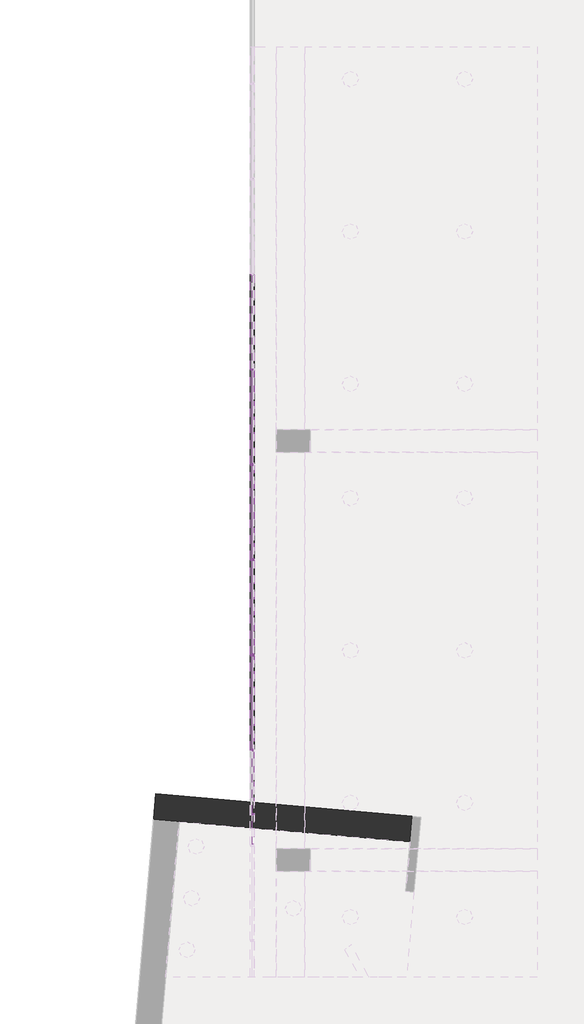
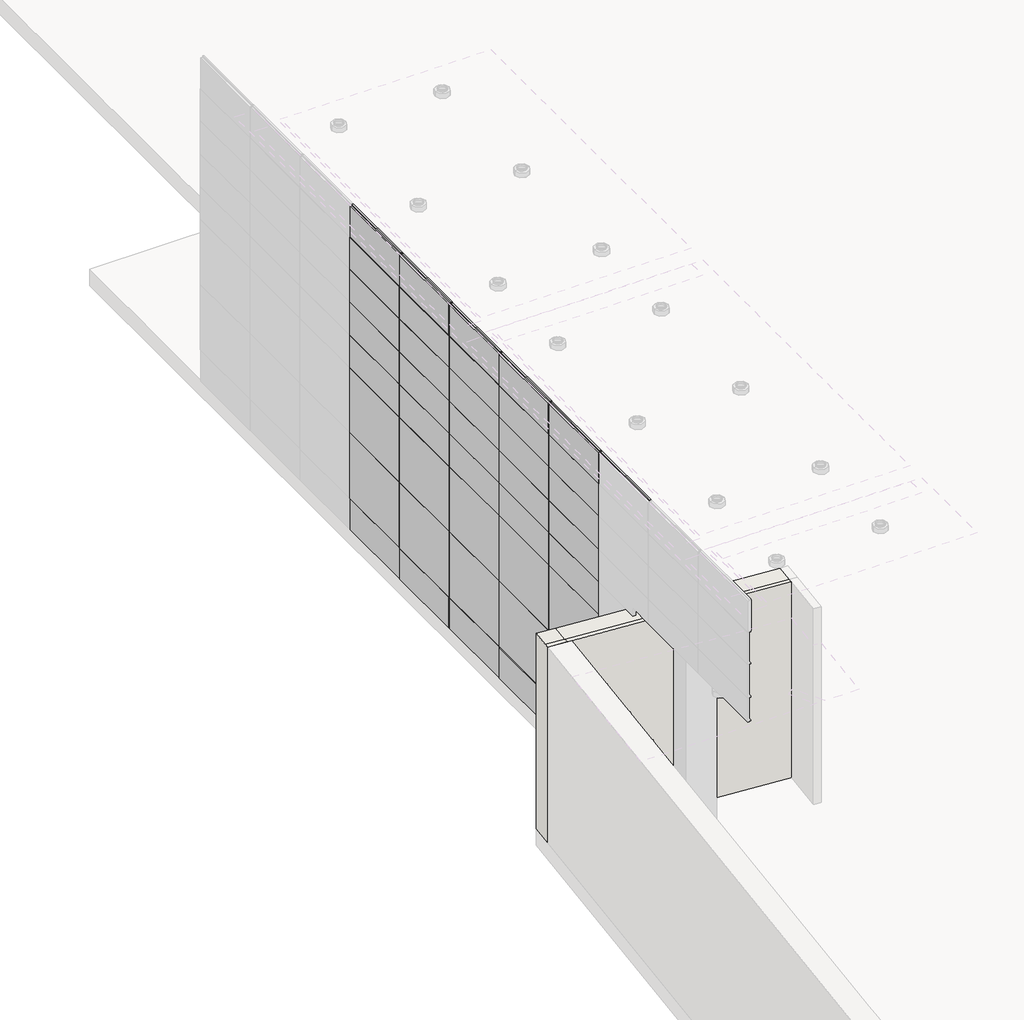
# One storey, part 6 of 30: 90 members, 40 plates, 1 wall.
"""IFC4 building model written with IfcOpenShell, lengths in millimetres."""

import ifcopenshell
import ifcopenshell.guid

model = None  # the IFC model being written
_history = None  # IfcOwnerHistory: only IFC2X3 demands one
_inside = {}  # id of a spatial element -> (the spatial element, [elements in it])
_under = {}  # id of a project, library or spatial element -> (it, [spatial elements below it])
_declared = {}  # id of a project -> (the project, [libraries it declares])
_typed = {}  # id of a type object -> (the type object, [elements of that type])
_made_of = {}  # id of a material, layer set ... -> (it, [elements and type objects made of it])


def new_model(schema):
    """Start an empty IFC model of exactly this schema.

    Asked for "IFC4X3", IfcOpenShell would pick the latest addendum, in which some entities
    have other attributes; the version numbers below select the first issue.
    IFC2X3 requires an IfcOwnerHistory on every rooted entity: one is made here for all.
    """
    global model, _history
    if schema == "IFC4X3":
        model = ifcopenshell.file(schema_version=(4, 3, 0, 0))
    else:
        model = ifcopenshell.file(schema=schema)
    _inside.clear()
    _under.clear()
    _declared.clear()
    _typed.clear()
    _made_of.clear()
    _history = None
    if model.schema == "IFC2X3":
        org = make("IfcOrganization", Name="unknown")
        user = make(
            "IfcPersonAndOrganization",
            ThePerson=make("IfcPerson", FamilyName="unknown"),
            TheOrganization=org,
        )
        app = make(
            "IfcApplication",
            ApplicationDeveloper=org,
            Version="unknown",
            ApplicationFullName="unknown",
            ApplicationIdentifier="unknown",
        )
        _history = make(
            "IfcOwnerHistory",
            OwningUser=user,
            OwningApplication=app,
            ChangeAction="ADDED",
            CreationDate=0,
        )
    return model


def make(cls, **values):
    """One entity of the class cls with the attributes given. An attribute that is None is left unset."""
    return model.create_entity(
        cls, **{name: value for name, value in values.items() if value is not None}
    )


def rooted(cls, **values):
    """An entity with a GlobalId (a new one), such as an element, a storey or a relation."""
    return make(cls, GlobalId=ifcopenshell.guid.new(), OwnerHistory=_history, **values)


def si_unit(unit_type, name, prefix=None):
    """IfcSIUnit, for example si_unit("LENGTHUNIT", "METRE", prefix="MILLI")."""
    return make("IfcSIUnit", UnitType=unit_type, Prefix=prefix, Name=name)


def assignment(units):
    """IfcUnitAssignment: the units of a project."""
    return None if units is None else make("IfcUnitAssignment", Units=units)


def point(xyz):
    """IfcCartesianPoint."""
    return None if xyz is None else make("IfcCartesianPoint", Coordinates=xyz)


def direction(xyz):
    """IfcDirection."""
    return None if xyz is None else make("IfcDirection", DirectionRatios=xyz)


def frame(location, z_axis=None, x_axis=None):
    """IfcAxis2Placement3D, a coordinate frame: its origin and axes. An axis left out is left unset."""
    return make(
        "IfcAxis2Placement3D",
        Location=point(location),
        Axis=direction(z_axis),
        RefDirection=direction(x_axis),
    )


def origin():
    """The frame at (0, 0, 0) with its axes left unset."""
    return frame((0.0, 0.0, 0.0))


def origin_with_axes():
    """The frame at (0, 0, 0) with the z axis (0, 0, 1) and the x axis (1, 0, 0) written out."""
    return frame((0.0, 0.0, 0.0), z_axis=(0.0, 0.0, 1.0), x_axis=(1.0, 0.0, 0.0))


def place(relative_to, where):
    """IfcLocalPlacement: puts the frame where relative to a parent placement (None: the world)."""
    return make(
        "IfcLocalPlacement", PlacementRelTo=relative_to, RelativePlacement=where
    )


def context(
    kind, dimensions, precision=None, world=None, true_north=None, identifier=None
):
    """IfcGeometricRepresentationContext, for example the 3D "Model" context."""
    return make(
        "IfcGeometricRepresentationContext",
        ContextIdentifier=identifier,
        ContextType=kind,
        CoordinateSpaceDimension=dimensions,
        Precision=precision,
        WorldCoordinateSystem=world,
        TrueNorth=true_north,
    )


def project(units=None, contexts=None):
    """IfcProject with its units and contexts."""
    return rooted(
        "IfcProject",
        Name="project",
        RepresentationContexts=contexts,
        UnitsInContext=assignment(units),
    )


def spatial(cls, under=None, at=None, **own):
    """A site, building, storey or space (cls), placed at a placement, below another one or the project."""
    s = rooted(cls, ObjectPlacement=at, **own)
    if under is not None:
        _under.setdefault(under.id(), (under, []))[1].append(s)
    return s


def polyline(points):
    """IfcPolyline through the points."""
    return make("IfcPolyline", Points=[point(p) for p in points])


def outline(outer, holes=None, kind="AREA"):
    """IfcArbitraryClosedProfileDef: a profile drawn as a closed curve; with holes, ...WithVoids."""
    if holes is None:
        return make("IfcArbitraryClosedProfileDef", ProfileType=kind, OuterCurve=outer)
    return make(
        "IfcArbitraryProfileDefWithVoids",
        ProfileType=kind,
        OuterCurve=outer,
        InnerCurves=holes,
    )


def extrude(swept, where, along, depth):
    """IfcExtrudedAreaSolid: the profile swept, set in the frame where, extruded along a direction by depth."""
    return make(
        "IfcExtrudedAreaSolid",
        SweptArea=swept,
        Position=where,
        ExtrudedDirection=direction(along),
        Depth=depth,
    )


def faces_of(points, faces, orient=None, outer=None):
    """IfcFace entities. A face is a list of loops; a loop is a list of indices into points, from 0.

    orient and outer hold one flag for each loop. By default every Orientation is true, the
    first loop of a face is its IfcFaceOuterBound and the others are IfcFaceBound.
    """
    made = []
    for i, loops in enumerate(faces):
        bounds = []
        for j, loop in enumerate(loops):
            is_outer = j == 0 if outer is None else outer[i][j]
            bounds.append(
                make(
                    "IfcFaceOuterBound" if is_outer else "IfcFaceBound",
                    Bound=make("IfcPolyLoop", Polygon=[points[k] for k in loop]),
                    Orientation=True if orient is None else orient[i][j],
                )
            )
        made.append(make("IfcFace", Bounds=bounds))
    return made


def faceted_brep(points, faces, orient=None, outer=None, voids=None):
    """IfcFacetedBrep: a solid bounded by flat faces; with voids (closed shells), ...WithVoids."""
    shared = [point(p) for p in points]
    hull = make("IfcClosedShell", CfsFaces=faces_of(shared, faces, orient, outer))
    if voids is None:
        return make("IfcFacetedBrep", Outer=hull)
    return make(
        "IfcFacetedBrepWithVoids",
        Outer=hull,
        Voids=[
            make(cls, CfsFaces=faces_of(shared, fs, o, b)) for cls, fs, o, b in voids
        ],
    )


def shape(context_of_items, identifier, shape_type, items):
    """IfcShapeRepresentation: the items that make up one representation, for example the "Body"."""
    return make(
        "IfcShapeRepresentation",
        ContextOfItems=context_of_items,
        RepresentationIdentifier=identifier,
        RepresentationType=shape_type,
        Items=items,
    )


def source(mapping_origin, context_of_items, identifier, shape_type, items):
    """IfcRepresentationMap: a shape defined once, which mapped items show again and again."""
    return make(
        "IfcRepresentationMap",
        MappingOrigin=mapping_origin,
        MappedRepresentation=shape(context_of_items, identifier, shape_type, items),
    )


def transform(
    local_origin,
    x_axis=None,
    y_axis=None,
    z_axis=None,
    scale=None,
    scale2=None,
    scale3=None,
    uniform=True,
):
    """IfcCartesianTransformationOperator3D, or its non-uniform kind. x_axis, y_axis, z_axis: its Axis1, 2, 3."""
    if uniform:
        return make(
            "IfcCartesianTransformationOperator3D",
            Axis1=direction(x_axis),
            Axis2=direction(y_axis),
            LocalOrigin=point(local_origin),
            Scale=scale,
            Axis3=direction(z_axis),
        )
    return make(
        "IfcCartesianTransformationOperator3DnonUniform",
        Axis1=direction(x_axis),
        Axis2=direction(y_axis),
        LocalOrigin=point(local_origin),
        Scale=scale,
        Axis3=direction(z_axis),
        Scale2=scale2,
        Scale3=scale3,
    )


def mapped(mapping_source, mapping_target):
    """IfcMappedItem: shows the shape of a source again, moved by a transform."""
    return make(
        "IfcMappedItem", MappingSource=mapping_source, MappingTarget=mapping_target
    )


def made_of(thing, what):
    """Note that an element or type object is made of a material, layer set ...; save() writes the relation."""
    if what is not None:
        _made_of.setdefault(what.id(), (what, []))[1].append(thing)
    return thing


def element(
    cls,
    number,
    at=None,
    inside=None,
    cuts=None,
    type_object=None,
    material=None,
    context=None,
    identifier="Body",
    shape_type=None,
    held_by="IfcProductDefinitionShape",
    body=None,
    shapes=None,
    **own,
):
    """One element of the class cls, such as IfcWall. Its Tag is "e" and its number.

    at: its placement. inside: the storey or other place that contains it. cuts: it is an
    opening in that element (IfcRelVoidsElement). A single representation is given by context,
    identifier, shape_type and body (its items); several are given by shapes. held_by: the class
    of the entity that holds the representations. save() writes the other relations.
    """
    e = rooted(cls, Tag="e%d" % number, ObjectPlacement=at, **own)
    if body is not None:
        shapes = [shape(context, identifier, shape_type, body)]
    if shapes is not None:
        e.Representation = make(held_by, Representations=shapes)
    if inside is not None:
        _inside.setdefault(inside.id(), (inside, []))[1].append(e)
    if cuts is not None:
        rooted(
            "IfcRelVoidsElement", RelatingBuildingElement=cuts, RelatedOpeningElement=e
        )
    if type_object is not None:
        _typed.setdefault(type_object.id(), (type_object, []))[1].append(e)
    return made_of(e, material)


def aggregate(whole, parts):
    """IfcRelAggregates: a whole, such as a stair, and the parts it consists of."""
    return rooted("IfcRelAggregates", RelatingObject=whole, RelatedObjects=parts)


def save(model, path):
    """Write the relations noted so far, then the file.

    IfcRelAggregates (storeys below a building ...), IfcRelContainedInSpatialStructure (elements
    in a storey), IfcRelDefinesByType, IfcRelAssociatesMaterial and IfcRelDeclares: one each for
    every whole, place, type object, material and project.
    """
    for whole, parts in _under.values():
        aggregate(whole, parts)
    for where, things in _inside.values():
        rooted(
            "IfcRelContainedInSpatialStructure",
            RelatedElements=things,
            RelatingStructure=where,
        )
    for kind, things in _typed.values():
        rooted("IfcRelDefinesByType", RelatedObjects=things, RelatingType=kind)
    for what, things in _made_of.values():
        rooted("IfcRelAssociatesMaterial", RelatedObjects=things, RelatingMaterial=what)
    for by, libraries in _declared.values():
        rooted("IfcRelDeclares", RelatingContext=by, RelatedDefinitions=libraries)
    model.write(path)


def member_f4845628(model_context):
    return source(origin(), model_context, "Body", "SweptSolid", [
        extrude(outline(polyline([(12.7, 12.7), (12.7, -12.7), (-12.7, -12.7), (-12.7, 12.7), (12.7, 12.7)])), frame((0.0, 0.0, -1219.2), z_axis=(0.0, 0.0, 1.0), x_axis=(1.0, 0.0, 0.0)), (0.0, 0.0, 1.0), 1219.2),
    ])


def member_6604d1e0(model_context):
    return source(origin(), model_context, "Body", "SweptSolid", [
        extrude(outline(polyline([(0.0, 12.7), (0.0, -12.7), (-25.4, -12.7), (-25.4, 12.7), (0.0, 12.7)])), frame((0.0, 0.0, -1498.6), z_axis=(0.0, 0.0, 1.0), x_axis=(1.0, 0.0, 0.0)), (0.0, 0.0, 1.0), 1498.6),
    ])


def member_68981e21(model_context):
    return source(origin(), model_context, "Body", "SweptSolid", [
        extrude(outline(polyline([(0.0, 12.7), (0.0, -12.7), (-25.4, -12.7), (-25.4, 12.7), (0.0, 12.7)])), frame((0.0, 0.0, -609.6), z_axis=(0.0, 0.0, 1.0), x_axis=(1.0, 0.0, 0.0)), (0.0, 0.0, 1.0), 609.6),
    ])


def member_9fd3d903(model_context):
    return source(origin(), model_context, "Body", "SweptSolid", [
        extrude(outline(polyline([(12.7, 12.7), (12.7, -12.7), (-12.7, -12.7), (-12.7, 12.7), (12.7, 12.7)])), frame((0.0, 0.0, -1498.6), z_axis=(0.0, 0.0, 1.0), x_axis=(1.0, 0.0, 0.0)), (0.0, 0.0, 1.0), 1498.6),
    ])


def member_3e1f1dd8(model_context):
    return source(origin(), model_context, "Body", "SweptSolid", [
        extrude(outline(polyline([(12.7, 12.7), (12.7, -12.7), (-12.7, -12.7), (-12.7, 12.7), (12.7, 12.7)])), frame((0.0, 0.0, -609.6), z_axis=(0.0, 0.0, 1.0), x_axis=(1.0, 0.0, 0.0)), (0.0, 0.0, 1.0), 609.6),
    ])


def member_93cf2621(model_context):
    return source(origin(), model_context, "Body", "SweptSolid", [
        extrude(outline(polyline([(12.7, 12.7), (12.7, -12.7), (-12.7, -12.7), (-12.7, 12.7), (12.7, 12.7)])), frame((0.0, 0.0, -622.3), z_axis=(0.0, 0.0, 1.0), x_axis=(1.0, 0.0, 0.0)), (0.0, 0.0, 1.0), 622.3),
    ])


def member_0acad92b(model_context):
    return source(origin(), model_context, "Body", "SweptSolid", [
        extrude(outline(polyline([(12.7, 12.7), (12.7, -12.7), (-12.7, -12.7), (-12.7, 12.7), (12.7, 12.7)])), frame((0.0, 0.0, -596.9), z_axis=(0.0, 0.0, 1.0), x_axis=(1.0, 0.0, 0.0)), (0.0, 0.0, 1.0), 596.9),
    ])


def member_b874cca0(model_context):
    return source(origin(), model_context, "Body", "SweptSolid", [
        extrude(outline(polyline([(12.7, 12.7), (12.7, -12.7), (-12.7, -12.7), (-12.7, 12.7), (12.7, 12.7)])), frame((0.0, 0.0, -1004.9287927), z_axis=(0.0, 0.0, 1.0), x_axis=(1.0, 0.0, 0.0)), (0.0, 0.0, 1.0), 1004.9287927),
    ])


def system_panel_glazed_327285c7(model_context):
    return source(origin(), model_context, "Body", "SweptSolid", [
        extrude(outline(polyline([(762.0, 19.05), (-762.0, 19.05), (-762.0, 44.45), (762.0, 44.45), (762.0, 19.05)])), origin_with_axes(), (0.0, 0.0, 1.0), 609.6),
    ])


def system_panel_glazed_14200f5a(model_context):
    return source(origin(), model_context, "Body", "SweptSolid", [
        extrude(outline(polyline([(762.0, 19.05), (-762.0, 19.05), (-762.0, 44.45), (762.0, 44.45), (762.0, 19.05)])), origin_with_axes(), (0.0, 0.0, 1.0), 1219.2),
    ])


def system_panel_glazed_39099b5e(model_context):
    return source(origin(), model_context, "Body", "SweptSolid", [
        extrude(outline(polyline([(762.0, 19.05), (-762.0, 19.05), (-762.0, 44.45), (762.0, 44.45), (762.0, 19.05)])), origin_with_axes(), (0.0, 0.0, 1.0), 622.3),
    ])


def system_panel_glazed_72237fa4(model_context):
    return source(origin(), model_context, "Body", "SweptSolid", [
        extrude(outline(polyline([(762.0, 19.05), (-762.0, 19.05), (-762.0, 44.45), (762.0, 44.45), (762.0, 19.05)])), origin_with_axes(), (0.0, 0.0, 1.0), 596.9),
    ])


def system_panel_solid_1afbd22d(model_context):
    return source(origin(), model_context, "Body", "SweptSolid", [
        extrude(outline(polyline([(749.3, -19.05), (-749.3, -19.05), (-749.3, 44.45), (749.3, 44.45), (749.3, -19.05)])), origin_with_axes(), (0.0, 0.0, 1.0), 571.5),
    ])


model = new_model("IFC4")

# Units and contexts
model_context = context("Model", 3, world=origin())
ifc_project = project(units=[si_unit("LENGTHUNIT", "METRE", prefix="MILLI")], contexts=[model_context])

# Site, building, storey
site = spatial("IfcSite", under=ifc_project)
building = spatial("IfcBuilding", under=site)
storey = spatial("IfcBuildingStorey", under=building, Name="1ST. FL.", Elevation=0.0)

# Members
placement = place(None, origin())
member_shape = member_f4845628(model_context)
element("IfcMember", 1, ObjectType="Rectangular Mullion : 1\" Square", at=placement, inside=storey, context=model_context, shape_type="MappedRepresentation", body=[
    mapped(member_shape, transform((-52109.6440345, -10845.0096347, 609.6), x_axis=(0.0, 1.0, 0.0), y_axis=(1.0, 0.0, 0.0), z_axis=(0.0, 0.0, -1.0))),
])
element("IfcMember", 2, ObjectType="Rectangular Mullion : 1\" Square", at=placement, inside=storey, context=model_context, shape_type="MappedRepresentation", body=[
    mapped(member_shape, transform((-52109.6440345, -10845.0096347, 1828.8), x_axis=(0.0, 1.0, 0.0), y_axis=(1.0, 0.0, 0.0), z_axis=(0.0, 0.0, -1.0))),
])
element("IfcMember", 3, ObjectType="Rectangular Mullion : 1\" Square", at=placement, inside=storey, context=model_context, shape_type="MappedRepresentation", body=[
    mapped(member_shape, transform((-52109.6440345, -9321.0096347, 609.6), x_axis=(0.0, 1.0, 0.0), y_axis=(1.0, 0.0, 0.0), z_axis=(0.0, 0.0, -1.0))),
])
element("IfcMember", 4, ObjectType="Rectangular Mullion : 1\" Square", at=placement, inside=storey, context=model_context, shape_type="MappedRepresentation", body=[
    mapped(member_shape, transform((-52109.6440345, -7797.0096347, 609.6), x_axis=(0.0, 1.0, 0.0), y_axis=(1.0, 0.0, 0.0), z_axis=(0.0, 0.0, -1.0))),
])
element("IfcMember", 5, ObjectType="Rectangular Mullion : 1\" Square", at=placement, inside=storey, context=model_context, shape_type="MappedRepresentation", body=[
    mapped(member_shape, transform((-52109.6440345, -6273.0096347, 609.6), x_axis=(0.0, 1.0, 0.0), y_axis=(1.0, 0.0, 0.0), z_axis=(0.0, 0.0, -1.0))),
])
element("IfcMember", 6, ObjectType="Rectangular Mullion : 1\" Square", at=placement, inside=storey, context=model_context, shape_type="MappedRepresentation", body=[
    mapped(member_shape, transform((-52109.6440345, -4749.0096347, 609.6), x_axis=(0.0, 1.0, 0.0), y_axis=(1.0, 0.0, 0.0), z_axis=(0.0, 0.0, -1.0))),
])
element("IfcMember", 7, ObjectType="Rectangular Mullion : 1\" Square", at=placement, inside=storey, context=model_context, shape_type="MappedRepresentation", body=[
    mapped(member_shape, transform((-52109.6440345, -9321.0096347, 1828.8), x_axis=(0.0, 1.0, 0.0), y_axis=(1.0, 0.0, 0.0), z_axis=(0.0, 0.0, -1.0))),
])
element("IfcMember", 8, ObjectType="Rectangular Mullion : 1\" Square", at=placement, inside=storey, context=model_context, shape_type="MappedRepresentation", body=[
    mapped(member_shape, transform((-52109.6440345, -7797.0096347, 1828.8), x_axis=(0.0, 1.0, 0.0), y_axis=(1.0, 0.0, 0.0), z_axis=(0.0, 0.0, -1.0))),
])
element("IfcMember", 9, ObjectType="Rectangular Mullion : 1\" Square", at=placement, inside=storey, context=model_context, shape_type="MappedRepresentation", body=[
    mapped(member_shape, transform((-52109.6440345, -6273.0096347, 1828.8), x_axis=(0.0, 1.0, 0.0), y_axis=(1.0, 0.0, 0.0), z_axis=(0.0, 0.0, -1.0))),
])
element("IfcMember", 10, ObjectType="Rectangular Mullion : 1\" Square", at=placement, inside=storey, context=model_context, shape_type="MappedRepresentation", body=[
    mapped(member_shape, transform((-52109.6440345, -4749.0096347, 1828.8), x_axis=(0.0, 1.0, 0.0), y_axis=(1.0, 0.0, 0.0), z_axis=(0.0, 0.0, -1.0))),
])
member_2_shape = member_6604d1e0(model_context)
element("IfcMember", 11, ObjectType="Rectangular Mullion : 1\" Square", at=placement, inside=storey, context=model_context, shape_type="MappedRepresentation", body=[
    mapped(member_2_shape, transform((-52109.6440345, -10857.7096347, 6096.0), x_axis=(0.0, 0.0, 1.0), y_axis=(1.0, 0.0, 0.0), z_axis=(0.0, 1.0, 0.0))),
])
element("IfcMember", 12, ObjectType="Rectangular Mullion : 1\" Square", at=placement, inside=storey, context=model_context, shape_type="MappedRepresentation", body=[
    mapped(member_2_shape, transform((-52109.6440345, -9333.7096347, 6096.0), x_axis=(0.0, 0.0, 1.0), y_axis=(1.0, 0.0, 0.0), z_axis=(0.0, 1.0, 0.0))),
])
element("IfcMember", 13, ObjectType="Rectangular Mullion : 1\" Square", at=placement, inside=storey, context=model_context, shape_type="MappedRepresentation", body=[
    mapped(member_2_shape, transform((-52109.6440345, -7809.7096347, 6096.0), x_axis=(0.0, 0.0, 1.0), y_axis=(1.0, 0.0, 0.0), z_axis=(0.0, 1.0, 0.0))),
])
element("IfcMember", 14, ObjectType="Rectangular Mullion : 1\" Square", at=placement, inside=storey, context=model_context, shape_type="MappedRepresentation", body=[
    mapped(member_2_shape, transform((-52109.6440345, -6285.7096347, 6096.0), x_axis=(0.0, 0.0, 1.0), y_axis=(1.0, 0.0, 0.0), z_axis=(0.0, 1.0, 0.0))),
])
element("IfcMember", 15, ObjectType="Rectangular Mullion : 1\" Square", at=placement, inside=storey, context=model_context, shape_type="MappedRepresentation", body=[
    mapped(member_2_shape, transform((-52109.6440345, -4761.7096347, 6096.0), x_axis=(0.0, 0.0, 1.0), y_axis=(1.0, 0.0, 0.0), z_axis=(0.0, 1.0, 0.0))),
])
element("IfcMember", 16, ObjectType="Rectangular Mullion : 1\" Square", at=placement, inside=storey, context=model_context, shape_type="MappedRepresentation", body=[
    mapped(member_2_shape, transform((-52109.6440345, -3237.7096347, 6096.0), x_axis=(0.0, 0.0, 1.0), y_axis=(1.0, 0.0, 0.0), z_axis=(0.0, 1.0, 0.0))),
])
element("IfcMember", 17, ObjectType="Rectangular Mullion : 1\" Square", at=placement, inside=storey, context=model_context, shape_type="MappedRepresentation", body=[
    mapped(member_2_shape, transform((-52109.6440345, -10832.3096347, 0.0), x_axis=(0.0, 0.0, -1.0), y_axis=(1.0, 0.0, 0.0), z_axis=(0.0, -1.0, 0.0))),
])
element("IfcMember", 18, ObjectType="Rectangular Mullion : 1\" Square", at=placement, inside=storey, context=model_context, shape_type="MappedRepresentation", body=[
    mapped(member_2_shape, transform((-52109.6440345, -9308.3096347, 0.0), x_axis=(0.0, 0.0, -1.0), y_axis=(1.0, 0.0, 0.0), z_axis=(0.0, -1.0, 0.0))),
])
element("IfcMember", 19, ObjectType="Rectangular Mullion : 1\" Square", at=placement, inside=storey, context=model_context, shape_type="MappedRepresentation", body=[
    mapped(member_2_shape, transform((-52109.6440345, -7784.3096347, 0.0), x_axis=(0.0, 0.0, -1.0), y_axis=(1.0, 0.0, 0.0), z_axis=(0.0, -1.0, 0.0))),
])
element("IfcMember", 20, ObjectType="Rectangular Mullion : 1\" Square", at=placement, inside=storey, context=model_context, shape_type="MappedRepresentation", body=[
    mapped(member_2_shape, transform((-52109.6440345, -6260.3096347, 0.0), x_axis=(0.0, 0.0, -1.0), y_axis=(1.0, 0.0, 0.0), z_axis=(0.0, -1.0, 0.0))),
])
element("IfcMember", 21, ObjectType="Rectangular Mullion : 1\" Square", at=placement, inside=storey, context=model_context, shape_type="MappedRepresentation", body=[
    mapped(member_2_shape, transform((-52109.6440345, -4736.3096347, 0.0), x_axis=(0.0, 0.0, -1.0), y_axis=(1.0, 0.0, 0.0), z_axis=(0.0, -1.0, 0.0))),
])
element("IfcMember", 22, ObjectType="Rectangular Mullion : 1\" Square", at=placement, inside=storey, context=model_context, shape_type="MappedRepresentation", body=[
    mapped(member_2_shape, transform((-52109.6440345, -3212.3096347, 0.0), x_axis=(0.0, 0.0, -1.0), y_axis=(1.0, 0.0, 0.0), z_axis=(0.0, -1.0, 0.0))),
])
member_3_shape = member_68981e21(model_context)
element("IfcMember", 23, ObjectType="Rectangular Mullion : 1\" Square", at=placement, inside=storey, context=model_context, shape_type="MappedRepresentation", body=[
    mapped(member_3_shape, transform((-52109.6440345, -11888.0384274, 3657.6), x_axis=(0.0, -1.0, 0.0), y_axis=(1.0, 0.0, 0.0), z_axis=(0.0, 0.0, 1.0))),
])
member_4_shape = member_9fd3d903(model_context)
element("IfcMember", 24, ObjectType="Rectangular Mullion : 1\" Square", at=placement, inside=storey, context=model_context, shape_type="MappedRepresentation", body=[
    mapped(member_4_shape, transform((-52109.6440345, -9333.7096347, 609.6), x_axis=(0.0, 0.0, 1.0), y_axis=(1.0, 0.0, 0.0), z_axis=(0.0, 1.0, 0.0))),
])
element("IfcMember", 25, ObjectType="Rectangular Mullion : 1\" Square", at=placement, inside=storey, context=model_context, shape_type="MappedRepresentation", body=[
    mapped(member_4_shape, transform((-52109.6440345, -9333.7096347, 1828.8), x_axis=(0.0, 0.0, 1.0), y_axis=(1.0, 0.0, 0.0), z_axis=(0.0, 1.0, 0.0))),
])
element("IfcMember", 26, ObjectType="Rectangular Mullion : 1\" Square", at=placement, inside=storey, context=model_context, shape_type="MappedRepresentation", body=[
    mapped(member_4_shape, transform((-52109.6440345, -9333.7096347, 3048.0), x_axis=(0.0, 0.0, 1.0), y_axis=(1.0, 0.0, 0.0), z_axis=(0.0, 1.0, 0.0))),
])
element("IfcMember", 27, ObjectType="Rectangular Mullion : 1\" Square", at=placement, inside=storey, context=model_context, shape_type="MappedRepresentation", body=[
    mapped(member_4_shape, transform((-52109.6440345, -9333.7096347, 3657.6), x_axis=(0.0, 0.0, 1.0), y_axis=(1.0, 0.0, 0.0), z_axis=(0.0, 1.0, 0.0))),
])
element("IfcMember", 28, ObjectType="Rectangular Mullion : 1\" Square", at=placement, inside=storey, context=model_context, shape_type="MappedRepresentation", body=[
    mapped(member_4_shape, transform((-52109.6440345, -10857.7096347, 4267.2), x_axis=(0.0, 0.0, 1.0), y_axis=(1.0, 0.0, 0.0), z_axis=(0.0, 1.0, 0.0))),
])
element("IfcMember", 29, ObjectType="Rectangular Mullion : 1\" Square", at=placement, inside=storey, context=model_context, shape_type="MappedRepresentation", body=[
    mapped(member_4_shape, transform((-52109.6440345, -9333.7096347, 4267.2), x_axis=(0.0, 0.0, 1.0), y_axis=(1.0, 0.0, 0.0), z_axis=(0.0, 1.0, 0.0))),
])
element("IfcMember", 30, ObjectType="Rectangular Mullion : 1\" Square", at=placement, inside=storey, context=model_context, shape_type="MappedRepresentation", body=[
    mapped(member_4_shape, transform((-52109.6440345, -10857.7096347, 4889.5), x_axis=(0.0, 0.0, 1.0), y_axis=(1.0, 0.0, 0.0), z_axis=(0.0, 1.0, 0.0))),
])
element("IfcMember", 31, ObjectType="Rectangular Mullion : 1\" Square", at=placement, inside=storey, context=model_context, shape_type="MappedRepresentation", body=[
    mapped(member_4_shape, transform((-52109.6440345, -9333.7096347, 4889.5), x_axis=(0.0, 0.0, 1.0), y_axis=(1.0, 0.0, 0.0), z_axis=(0.0, 1.0, 0.0))),
])
element("IfcMember", 32, ObjectType="Rectangular Mullion : 1\" Square", at=placement, inside=storey, context=model_context, shape_type="MappedRepresentation", body=[
    mapped(member_4_shape, transform((-52109.6440345, -10857.7096347, 5486.4), x_axis=(0.0, 0.0, 1.0), y_axis=(1.0, 0.0, 0.0), z_axis=(0.0, 1.0, 0.0))),
])
element("IfcMember", 33, ObjectType="Rectangular Mullion : 1\" Square", at=placement, inside=storey, context=model_context, shape_type="MappedRepresentation", body=[
    mapped(member_4_shape, transform((-52109.6440345, -9333.7096347, 5486.4), x_axis=(0.0, 0.0, 1.0), y_axis=(1.0, 0.0, 0.0), z_axis=(0.0, 1.0, 0.0))),
])
element("IfcMember", 34, ObjectType="Rectangular Mullion : 1\" Square", at=placement, inside=storey, context=model_context, shape_type="MappedRepresentation", body=[
    mapped(member_4_shape, transform((-52109.6440345, -7809.7096347, 609.6), x_axis=(0.0, 0.0, 1.0), y_axis=(1.0, 0.0, 0.0), z_axis=(0.0, 1.0, 0.0))),
])
element("IfcMember", 35, ObjectType="Rectangular Mullion : 1\" Square", at=placement, inside=storey, context=model_context, shape_type="MappedRepresentation", body=[
    mapped(member_4_shape, transform((-52109.6440345, -6285.7096347, 609.6), x_axis=(0.0, 0.0, 1.0), y_axis=(1.0, 0.0, 0.0), z_axis=(0.0, 1.0, 0.0))),
])
element("IfcMember", 36, ObjectType="Rectangular Mullion : 1\" Square", at=placement, inside=storey, context=model_context, shape_type="MappedRepresentation", body=[
    mapped(member_4_shape, transform((-52109.6440345, -4761.7096347, 609.6), x_axis=(0.0, 0.0, 1.0), y_axis=(1.0, 0.0, 0.0), z_axis=(0.0, 1.0, 0.0))),
])
element("IfcMember", 37, ObjectType="Rectangular Mullion : 1\" Square", at=placement, inside=storey, context=model_context, shape_type="MappedRepresentation", body=[
    mapped(member_4_shape, transform((-52109.6440345, -3237.7096347, 609.6), x_axis=(0.0, 0.0, 1.0), y_axis=(1.0, 0.0, 0.0), z_axis=(0.0, 1.0, 0.0))),
])
element("IfcMember", 38, ObjectType="Rectangular Mullion : 1\" Square", at=placement, inside=storey, context=model_context, shape_type="MappedRepresentation", body=[
    mapped(member_4_shape, transform((-52109.6440345, -7809.7096347, 1828.8), x_axis=(0.0, 0.0, 1.0), y_axis=(1.0, 0.0, 0.0), z_axis=(0.0, 1.0, 0.0))),
])
element("IfcMember", 39, ObjectType="Rectangular Mullion : 1\" Square", at=placement, inside=storey, context=model_context, shape_type="MappedRepresentation", body=[
    mapped(member_4_shape, transform((-52109.6440345, -6285.7096347, 1828.8), x_axis=(0.0, 0.0, 1.0), y_axis=(1.0, 0.0, 0.0), z_axis=(0.0, 1.0, 0.0))),
])
element("IfcMember", 40, ObjectType="Rectangular Mullion : 1\" Square", at=placement, inside=storey, context=model_context, shape_type="MappedRepresentation", body=[
    mapped(member_4_shape, transform((-52109.6440345, -4761.7096347, 1828.8), x_axis=(0.0, 0.0, 1.0), y_axis=(1.0, 0.0, 0.0), z_axis=(0.0, 1.0, 0.0))),
])
element("IfcMember", 41, ObjectType="Rectangular Mullion : 1\" Square", at=placement, inside=storey, context=model_context, shape_type="MappedRepresentation", body=[
    mapped(member_4_shape, transform((-52109.6440345, -3237.7096347, 1828.8), x_axis=(0.0, 0.0, 1.0), y_axis=(1.0, 0.0, 0.0), z_axis=(0.0, 1.0, 0.0))),
])
element("IfcMember", 42, ObjectType="Rectangular Mullion : 1\" Square", at=placement, inside=storey, context=model_context, shape_type="MappedRepresentation", body=[
    mapped(member_4_shape, transform((-52109.6440345, -7809.7096347, 3048.0), x_axis=(0.0, 0.0, 1.0), y_axis=(1.0, 0.0, 0.0), z_axis=(0.0, 1.0, 0.0))),
])
element("IfcMember", 43, ObjectType="Rectangular Mullion : 1\" Square", at=placement, inside=storey, context=model_context, shape_type="MappedRepresentation", body=[
    mapped(member_4_shape, transform((-52109.6440345, -6285.7096347, 3048.0), x_axis=(0.0, 0.0, 1.0), y_axis=(1.0, 0.0, 0.0), z_axis=(0.0, 1.0, 0.0))),
])
element("IfcMember", 44, ObjectType="Rectangular Mullion : 1\" Square", at=placement, inside=storey, context=model_context, shape_type="MappedRepresentation", body=[
    mapped(member_4_shape, transform((-52109.6440345, -4761.7096347, 3048.0), x_axis=(0.0, 0.0, 1.0), y_axis=(1.0, 0.0, 0.0), z_axis=(0.0, 1.0, 0.0))),
])
element("IfcMember", 45, ObjectType="Rectangular Mullion : 1\" Square", at=placement, inside=storey, context=model_context, shape_type="MappedRepresentation", body=[
    mapped(member_4_shape, transform((-52109.6440345, -7809.7096347, 3657.6), x_axis=(0.0, 0.0, 1.0), y_axis=(1.0, 0.0, 0.0), z_axis=(0.0, 1.0, 0.0))),
])
element("IfcMember", 46, ObjectType="Rectangular Mullion : 1\" Square", at=placement, inside=storey, context=model_context, shape_type="MappedRepresentation", body=[
    mapped(member_4_shape, transform((-52109.6440345, -6285.7096347, 3657.6), x_axis=(0.0, 0.0, 1.0), y_axis=(1.0, 0.0, 0.0), z_axis=(0.0, 1.0, 0.0))),
])
element("IfcMember", 47, ObjectType="Rectangular Mullion : 1\" Square", at=placement, inside=storey, context=model_context, shape_type="MappedRepresentation", body=[
    mapped(member_4_shape, transform((-52109.6440345, -4761.7096347, 3657.6), x_axis=(0.0, 0.0, 1.0), y_axis=(1.0, 0.0, 0.0), z_axis=(0.0, 1.0, 0.0))),
])
element("IfcMember", 48, ObjectType="Rectangular Mullion : 1\" Square", at=placement, inside=storey, context=model_context, shape_type="MappedRepresentation", body=[
    mapped(member_4_shape, transform((-52109.6440345, -7809.7096347, 4267.2), x_axis=(0.0, 0.0, 1.0), y_axis=(1.0, 0.0, 0.0), z_axis=(0.0, 1.0, 0.0))),
])
element("IfcMember", 49, ObjectType="Rectangular Mullion : 1\" Square", at=placement, inside=storey, context=model_context, shape_type="MappedRepresentation", body=[
    mapped(member_4_shape, transform((-52109.6440345, -6285.7096347, 4267.2), x_axis=(0.0, 0.0, 1.0), y_axis=(1.0, 0.0, 0.0), z_axis=(0.0, 1.0, 0.0))),
])
element("IfcMember", 50, ObjectType="Rectangular Mullion : 1\" Square", at=placement, inside=storey, context=model_context, shape_type="MappedRepresentation", body=[
    mapped(member_4_shape, transform((-52109.6440345, -4761.7096347, 4267.2), x_axis=(0.0, 0.0, 1.0), y_axis=(1.0, 0.0, 0.0), z_axis=(0.0, 1.0, 0.0))),
])
element("IfcMember", 51, ObjectType="Rectangular Mullion : 1\" Square", at=placement, inside=storey, context=model_context, shape_type="MappedRepresentation", body=[
    mapped(member_4_shape, transform((-52109.6440345, -7809.7096347, 4889.5), x_axis=(0.0, 0.0, 1.0), y_axis=(1.0, 0.0, 0.0), z_axis=(0.0, 1.0, 0.0))),
])
element("IfcMember", 52, ObjectType="Rectangular Mullion : 1\" Square", at=placement, inside=storey, context=model_context, shape_type="MappedRepresentation", body=[
    mapped(member_4_shape, transform((-52109.6440345, -6285.7096347, 4889.5), x_axis=(0.0, 0.0, 1.0), y_axis=(1.0, 0.0, 0.0), z_axis=(0.0, 1.0, 0.0))),
])
element("IfcMember", 53, ObjectType="Rectangular Mullion : 1\" Square", at=placement, inside=storey, context=model_context, shape_type="MappedRepresentation", body=[
    mapped(member_4_shape, transform((-52109.6440345, -4761.7096347, 4889.5), x_axis=(0.0, 0.0, 1.0), y_axis=(1.0, 0.0, 0.0), z_axis=(0.0, 1.0, 0.0))),
])
element("IfcMember", 54, ObjectType="Rectangular Mullion : 1\" Square", at=placement, inside=storey, context=model_context, shape_type="MappedRepresentation", body=[
    mapped(member_4_shape, transform((-52109.6440345, -7809.7096347, 5486.4), x_axis=(0.0, 0.0, 1.0), y_axis=(1.0, 0.0, 0.0), z_axis=(0.0, 1.0, 0.0))),
])
element("IfcMember", 55, ObjectType="Rectangular Mullion : 1\" Square", at=placement, inside=storey, context=model_context, shape_type="MappedRepresentation", body=[
    mapped(member_4_shape, transform((-52109.6440345, -6285.7096347, 5486.4), x_axis=(0.0, 0.0, 1.0), y_axis=(1.0, 0.0, 0.0), z_axis=(0.0, 1.0, 0.0))),
])
element("IfcMember", 56, ObjectType="Rectangular Mullion : 1\" Square", at=placement, inside=storey, context=model_context, shape_type="MappedRepresentation", body=[
    mapped(member_4_shape, transform((-52109.6440345, -4761.7096347, 5486.4), x_axis=(0.0, 0.0, 1.0), y_axis=(1.0, 0.0, 0.0), z_axis=(0.0, 1.0, 0.0))),
])
member_5_shape = member_3e1f1dd8(model_context)
element("IfcMember", 57, ObjectType="Rectangular Mullion : 1\" Square", at=placement, inside=storey, context=model_context, shape_type="MappedRepresentation", body=[
    mapped(member_5_shape, transform((-52109.6440345, -10845.0096347, 0.0), x_axis=(0.0, 1.0, 0.0), y_axis=(1.0, 0.0, 0.0), z_axis=(0.0, 0.0, -1.0))),
])
element("IfcMember", 58, ObjectType="Rectangular Mullion : 1\" Square", at=placement, inside=storey, context=model_context, shape_type="MappedRepresentation", body=[
    mapped(member_5_shape, transform((-52109.6440345, -9321.0096347, 0.0), x_axis=(0.0, 1.0, 0.0), y_axis=(1.0, 0.0, 0.0), z_axis=(0.0, 0.0, -1.0))),
])
element("IfcMember", 59, ObjectType="Rectangular Mullion : 1\" Square", at=placement, inside=storey, context=model_context, shape_type="MappedRepresentation", body=[
    mapped(member_5_shape, transform((-52109.6440345, -7797.0096347, 0.0), x_axis=(0.0, 1.0, 0.0), y_axis=(1.0, 0.0, 0.0), z_axis=(0.0, 0.0, -1.0))),
])
element("IfcMember", 60, ObjectType="Rectangular Mullion : 1\" Square", at=placement, inside=storey, context=model_context, shape_type="MappedRepresentation", body=[
    mapped(member_5_shape, transform((-52109.6440345, -6273.0096347, 0.0), x_axis=(0.0, 1.0, 0.0), y_axis=(1.0, 0.0, 0.0), z_axis=(0.0, 0.0, -1.0))),
])
element("IfcMember", 61, ObjectType="Rectangular Mullion : 1\" Square", at=placement, inside=storey, context=model_context, shape_type="MappedRepresentation", body=[
    mapped(member_5_shape, transform((-52109.6440345, -4749.0096347, 0.0), x_axis=(0.0, 1.0, 0.0), y_axis=(1.0, 0.0, 0.0), z_axis=(0.0, 0.0, -1.0))),
])
element("IfcMember", 62, ObjectType="Rectangular Mullion : 1\" Square", at=placement, inside=storey, context=model_context, shape_type="MappedRepresentation", body=[
    mapped(member_5_shape, transform((-52109.6440345, -10845.0096347, 3048.0), x_axis=(0.0, 1.0, 0.0), y_axis=(1.0, 0.0, 0.0), z_axis=(0.0, 0.0, -1.0))),
])
element("IfcMember", 63, ObjectType="Rectangular Mullion : 1\" Square", at=placement, inside=storey, context=model_context, shape_type="MappedRepresentation", body=[
    mapped(member_5_shape, transform((-52109.6440345, -10845.0096347, 3657.6), x_axis=(0.0, 1.0, 0.0), y_axis=(1.0, 0.0, 0.0), z_axis=(0.0, 0.0, -1.0))),
])
element("IfcMember", 64, ObjectType="Rectangular Mullion : 1\" Square", at=placement, inside=storey, context=model_context, shape_type="MappedRepresentation", body=[
    mapped(member_5_shape, transform((-52109.6440345, -9321.0096347, 3048.0), x_axis=(0.0, 1.0, 0.0), y_axis=(1.0, 0.0, 0.0), z_axis=(0.0, 0.0, -1.0))),
])
element("IfcMember", 65, ObjectType="Rectangular Mullion : 1\" Square", at=placement, inside=storey, context=model_context, shape_type="MappedRepresentation", body=[
    mapped(member_5_shape, transform((-52109.6440345, -7797.0096347, 3048.0), x_axis=(0.0, 1.0, 0.0), y_axis=(1.0, 0.0, 0.0), z_axis=(0.0, 0.0, -1.0))),
])
element("IfcMember", 66, ObjectType="Rectangular Mullion : 1\" Square", at=placement, inside=storey, context=model_context, shape_type="MappedRepresentation", body=[
    mapped(member_5_shape, transform((-52109.6440345, -6273.0096347, 3048.0), x_axis=(0.0, 1.0, 0.0), y_axis=(1.0, 0.0, 0.0), z_axis=(0.0, 0.0, -1.0))),
])
element("IfcMember", 67, ObjectType="Rectangular Mullion : 1\" Square", at=placement, inside=storey, context=model_context, shape_type="MappedRepresentation", body=[
    mapped(member_5_shape, transform((-52109.6440345, -4749.0096347, 3048.0), x_axis=(0.0, 1.0, 0.0), y_axis=(1.0, 0.0, 0.0), z_axis=(0.0, 0.0, -1.0))),
])
element("IfcMember", 68, ObjectType="Rectangular Mullion : 1\" Square", at=placement, inside=storey, context=model_context, shape_type="MappedRepresentation", body=[
    mapped(member_5_shape, transform((-52109.6440345, -9321.0096347, 3657.6), x_axis=(0.0, 1.0, 0.0), y_axis=(1.0, 0.0, 0.0), z_axis=(0.0, 0.0, -1.0))),
])
element("IfcMember", 69, ObjectType="Rectangular Mullion : 1\" Square", at=placement, inside=storey, context=model_context, shape_type="MappedRepresentation", body=[
    mapped(member_5_shape, transform((-52109.6440345, -7797.0096347, 3657.6), x_axis=(0.0, 1.0, 0.0), y_axis=(1.0, 0.0, 0.0), z_axis=(0.0, 0.0, -1.0))),
])
element("IfcMember", 70, ObjectType="Rectangular Mullion : 1\" Square", at=placement, inside=storey, context=model_context, shape_type="MappedRepresentation", body=[
    mapped(member_5_shape, transform((-52109.6440345, -6273.0096347, 3657.6), x_axis=(0.0, 1.0, 0.0), y_axis=(1.0, 0.0, 0.0), z_axis=(0.0, 0.0, -1.0))),
])
element("IfcMember", 71, ObjectType="Rectangular Mullion : 1\" Square", at=placement, inside=storey, context=model_context, shape_type="MappedRepresentation", body=[
    mapped(member_5_shape, transform((-52109.6440345, -4749.0096347, 3657.6), x_axis=(0.0, 1.0, 0.0), y_axis=(1.0, 0.0, 0.0), z_axis=(0.0, 0.0, -1.0))),
])
member_6_shape = member_93cf2621(model_context)
element("IfcMember", 72, ObjectType="Rectangular Mullion : 1\" Square", at=placement, inside=storey, context=model_context, shape_type="MappedRepresentation", body=[
    mapped(member_6_shape, transform((-52109.6440345, -10845.0096347, 4267.2), x_axis=(0.0, 1.0, 0.0), y_axis=(1.0, 0.0, 0.0), z_axis=(0.0, 0.0, -1.0))),
])
element("IfcMember", 73, ObjectType="Rectangular Mullion : 1\" Square", at=placement, inside=storey, context=model_context, shape_type="MappedRepresentation", body=[
    mapped(member_6_shape, transform((-52109.6440345, -9321.0096347, 4267.2), x_axis=(0.0, 1.0, 0.0), y_axis=(1.0, 0.0, 0.0), z_axis=(0.0, 0.0, -1.0))),
])
element("IfcMember", 74, ObjectType="Rectangular Mullion : 1\" Square", at=placement, inside=storey, context=model_context, shape_type="MappedRepresentation", body=[
    mapped(member_6_shape, transform((-52109.6440345, -7797.0096347, 4267.2), x_axis=(0.0, 1.0, 0.0), y_axis=(1.0, 0.0, 0.0), z_axis=(0.0, 0.0, -1.0))),
])
element("IfcMember", 75, ObjectType="Rectangular Mullion : 1\" Square", at=placement, inside=storey, context=model_context, shape_type="MappedRepresentation", body=[
    mapped(member_6_shape, transform((-52109.6440345, -6273.0096347, 4267.2), x_axis=(0.0, 1.0, 0.0), y_axis=(1.0, 0.0, 0.0), z_axis=(0.0, 0.0, -1.0))),
])
element("IfcMember", 76, ObjectType="Rectangular Mullion : 1\" Square", at=placement, inside=storey, context=model_context, shape_type="MappedRepresentation", body=[
    mapped(member_6_shape, transform((-52109.6440345, -4749.0096347, 4267.2), x_axis=(0.0, 1.0, 0.0), y_axis=(1.0, 0.0, 0.0), z_axis=(0.0, 0.0, -1.0))),
])
member_7_shape = member_0acad92b(model_context)
element("IfcMember", 77, ObjectType="Rectangular Mullion : 1\" Square", at=placement, inside=storey, context=model_context, shape_type="MappedRepresentation", body=[
    mapped(member_7_shape, transform((-52109.6440345, -10845.0096347, 4889.5), x_axis=(0.0, 1.0, 0.0), y_axis=(1.0, 0.0, 0.0), z_axis=(0.0, 0.0, -1.0))),
])
element("IfcMember", 78, ObjectType="Rectangular Mullion : 1\" Square", at=placement, inside=storey, context=model_context, shape_type="MappedRepresentation", body=[
    mapped(member_7_shape, transform((-52109.6440345, -9321.0096347, 4889.5), x_axis=(0.0, 1.0, 0.0), y_axis=(1.0, 0.0, 0.0), z_axis=(0.0, 0.0, -1.0))),
])
element("IfcMember", 79, ObjectType="Rectangular Mullion : 1\" Square", at=placement, inside=storey, context=model_context, shape_type="MappedRepresentation", body=[
    mapped(member_7_shape, transform((-52109.6440345, -7797.0096347, 4889.5), x_axis=(0.0, 1.0, 0.0), y_axis=(1.0, 0.0, 0.0), z_axis=(0.0, 0.0, -1.0))),
])
element("IfcMember", 80, ObjectType="Rectangular Mullion : 1\" Square", at=placement, inside=storey, context=model_context, shape_type="MappedRepresentation", body=[
    mapped(member_7_shape, transform((-52109.6440345, -6273.0096347, 4889.5), x_axis=(0.0, 1.0, 0.0), y_axis=(1.0, 0.0, 0.0), z_axis=(0.0, 0.0, -1.0))),
])
element("IfcMember", 81, ObjectType="Rectangular Mullion : 1\" Square", at=placement, inside=storey, context=model_context, shape_type="MappedRepresentation", body=[
    mapped(member_7_shape, transform((-52109.6440345, -4749.0096347, 4889.5), x_axis=(0.0, 1.0, 0.0), y_axis=(1.0, 0.0, 0.0), z_axis=(0.0, 0.0, -1.0))),
])
element("IfcMember", 82, ObjectType="Rectangular Mullion : 1\" Square", at=placement, inside=storey, context=model_context, shape_type="MappedRepresentation", body=[
    mapped(member_5_shape, transform((-52109.6440345, -10845.0096347, 5486.4), x_axis=(0.0, 1.0, 0.0), y_axis=(1.0, 0.0, 0.0), z_axis=(0.0, 0.0, -1.0))),
])
element("IfcMember", 83, ObjectType="Rectangular Mullion : 1\" Square", at=placement, inside=storey, context=model_context, shape_type="MappedRepresentation", body=[
    mapped(member_5_shape, transform((-52109.6440345, -9321.0096347, 5486.4), x_axis=(0.0, 1.0, 0.0), y_axis=(1.0, 0.0, 0.0), z_axis=(0.0, 0.0, -1.0))),
])
element("IfcMember", 84, ObjectType="Rectangular Mullion : 1\" Square", at=placement, inside=storey, context=model_context, shape_type="MappedRepresentation", body=[
    mapped(member_5_shape, transform((-52109.6440345, -7797.0096347, 5486.4), x_axis=(0.0, 1.0, 0.0), y_axis=(1.0, 0.0, 0.0), z_axis=(0.0, 0.0, -1.0))),
])
element("IfcMember", 85, ObjectType="Rectangular Mullion : 1\" Square", at=placement, inside=storey, context=model_context, shape_type="MappedRepresentation", body=[
    mapped(member_5_shape, transform((-52109.6440345, -6273.0096347, 5486.4), x_axis=(0.0, 1.0, 0.0), y_axis=(1.0, 0.0, 0.0), z_axis=(0.0, 0.0, -1.0))),
])
element("IfcMember", 86, ObjectType="Rectangular Mullion : 1\" Square", at=placement, inside=storey, context=model_context, shape_type="MappedRepresentation", body=[
    mapped(member_5_shape, transform((-52109.6440345, -4749.0096347, 5486.4), x_axis=(0.0, 1.0, 0.0), y_axis=(1.0, 0.0, 0.0), z_axis=(0.0, 0.0, -1.0))),
])
member_8_shape = member_b874cca0(model_context)
element("IfcMember", 87, ObjectType="Rectangular Mullion : 1\" Square", at=placement, inside=storey, context=model_context, shape_type="MappedRepresentation", body=[
    mapped(member_8_shape, transform((-52109.6440345, -10857.7096347, 609.6), x_axis=(0.0, 0.0, 1.0), y_axis=(1.0, 0.0, 0.0), z_axis=(0.0, 1.0, 0.0))),
])
element("IfcMember", 88, ObjectType="Rectangular Mullion : 1\" Square", at=placement, inside=storey, context=model_context, shape_type="MappedRepresentation", body=[
    mapped(member_8_shape, transform((-52109.6440345, -10857.7096347, 1828.8), x_axis=(0.0, 0.0, 1.0), y_axis=(1.0, 0.0, 0.0), z_axis=(0.0, 1.0, 0.0))),
])
element("IfcMember", 89, ObjectType="Rectangular Mullion : 1\" Square", at=placement, inside=storey, context=model_context, shape_type="MappedRepresentation", body=[
    mapped(member_8_shape, transform((-52109.6440345, -10857.7096347, 3048.0), x_axis=(0.0, 0.0, 1.0), y_axis=(1.0, 0.0, 0.0), z_axis=(0.0, 1.0, 0.0))),
])
element("IfcMember", 90, ObjectType="Rectangular Mullion : 1\" Square", at=placement, inside=storey, context=model_context, shape_type="MappedRepresentation", body=[
    mapped(member_8_shape, transform((-52109.6440345, -10857.7096347, 3657.6), x_axis=(0.0, 0.0, 1.0), y_axis=(1.0, 0.0, 0.0), z_axis=(0.0, 1.0, 0.0))),
])

# Plates
system_panel_glazed_shape = system_panel_glazed_327285c7(model_context)
element("IfcPlate", 91, ObjectType="System Panel : Glazed", at=placement, inside=storey, context=model_context, shape_type="MappedRepresentation", body=[
    mapped(system_panel_glazed_shape, transform((-52109.6440345, -10083.0096347, 3048.0), x_axis=(0.0, 1.0, 0.0), y_axis=(-1.0, 0.0, 0.0), z_axis=(0.0, 0.0, 1.0))),
])
element("IfcPlate", 92, ObjectType="System Panel : Glazed", at=placement, inside=storey, context=model_context, shape_type="MappedRepresentation", body=[
    mapped(system_panel_glazed_shape, transform((-52109.6440345, -10083.0096347, 3657.6), x_axis=(0.0, 1.0, 0.0), y_axis=(-1.0, 0.0, 0.0), z_axis=(0.0, 0.0, 1.0))),
])
element("IfcPlate", 93, ObjectType="System Panel : Glazed", at=placement, inside=storey, context=model_context, shape_type="MappedRepresentation", body=[
    mapped(system_panel_glazed_shape, transform((-52109.6440345, -8559.0096347, 3048.0), x_axis=(0.0, 1.0, 0.0), y_axis=(-1.0, 0.0, 0.0), z_axis=(0.0, 0.0, 1.0))),
])
element("IfcPlate", 94, ObjectType="System Panel : Glazed", at=placement, inside=storey, context=model_context, shape_type="MappedRepresentation", body=[
    mapped(system_panel_glazed_shape, transform((-52109.6440345, -8559.0096347, 3657.6), x_axis=(0.0, 1.0, 0.0), y_axis=(-1.0, 0.0, 0.0), z_axis=(0.0, 0.0, 1.0))),
])
element("IfcPlate", 95, ObjectType="System Panel : Glazed", at=placement, inside=storey, context=model_context, shape_type="MappedRepresentation", body=[
    mapped(system_panel_glazed_shape, transform((-52109.6440345, -7035.0096347, 3048.0), x_axis=(0.0, 1.0, 0.0), y_axis=(-1.0, 0.0, 0.0), z_axis=(0.0, 0.0, 1.0))),
])
element("IfcPlate", 96, ObjectType="System Panel : Glazed", at=placement, inside=storey, context=model_context, shape_type="MappedRepresentation", body=[
    mapped(system_panel_glazed_shape, transform((-52109.6440345, -7035.0096347, 3657.6), x_axis=(0.0, 1.0, 0.0), y_axis=(-1.0, 0.0, 0.0), z_axis=(0.0, 0.0, 1.0))),
])
element("IfcPlate", 97, ObjectType="System Panel : Glazed", at=placement, inside=storey, context=model_context, shape_type="MappedRepresentation", body=[
    mapped(system_panel_glazed_shape, transform((-52109.6440345, -5511.0096347, 3048.0), x_axis=(0.0, 1.0, 0.0), y_axis=(-1.0, 0.0, 0.0), z_axis=(0.0, 0.0, 1.0))),
])
element("IfcPlate", 98, ObjectType="System Panel : Glazed", at=placement, inside=storey, context=model_context, shape_type="MappedRepresentation", body=[
    mapped(system_panel_glazed_shape, transform((-52109.6440345, -5511.0096347, 3657.6), x_axis=(0.0, 1.0, 0.0), y_axis=(-1.0, 0.0, 0.0), z_axis=(0.0, 0.0, 1.0))),
])
element("IfcPlate", 99, ObjectType="System Panel : Glazed", at=placement, inside=storey, context=model_context, shape_type="MappedRepresentation", body=[
    mapped(system_panel_glazed_shape, transform((-52109.6440345, -3987.0096347, 3048.0), x_axis=(0.0, 1.0, 0.0), y_axis=(-1.0, 0.0, 0.0), z_axis=(0.0, 0.0, 1.0))),
])
element("IfcPlate", 100, ObjectType="System Panel : Glazed", at=placement, inside=storey, context=model_context, shape_type="MappedRepresentation", body=[
    mapped(system_panel_glazed_shape, transform((-52109.6440345, -3987.0096347, 3657.6), x_axis=(0.0, 1.0, 0.0), y_axis=(-1.0, 0.0, 0.0), z_axis=(0.0, 0.0, 1.0))),
])
system_panel_glazed_2_shape = system_panel_glazed_14200f5a(model_context)
element("IfcPlate", 101, ObjectType="System Panel : Glazed", at=placement, inside=storey, context=model_context, shape_type="MappedRepresentation", body=[
    mapped(system_panel_glazed_2_shape, transform((-52109.6440345, -10083.0096347, 609.6), x_axis=(0.0, 1.0, 0.0), y_axis=(-1.0, 0.0, 0.0), z_axis=(0.0, 0.0, 1.0))),
])
element("IfcPlate", 102, ObjectType="System Panel : Glazed", at=placement, inside=storey, context=model_context, shape_type="MappedRepresentation", body=[
    mapped(system_panel_glazed_2_shape, transform((-52109.6440345, -10083.0096347, 1828.8), x_axis=(0.0, 1.0, 0.0), y_axis=(-1.0, 0.0, 0.0), z_axis=(0.0, 0.0, 1.0))),
])
element("IfcPlate", 103, ObjectType="System Panel : Glazed", at=placement, inside=storey, context=model_context, shape_type="MappedRepresentation", body=[
    mapped(system_panel_glazed_2_shape, transform((-52109.6440345, -8559.0096347, 609.6), x_axis=(0.0, 1.0, 0.0), y_axis=(-1.0, 0.0, 0.0), z_axis=(0.0, 0.0, 1.0))),
])
element("IfcPlate", 104, ObjectType="System Panel : Glazed", at=placement, inside=storey, context=model_context, shape_type="MappedRepresentation", body=[
    mapped(system_panel_glazed_2_shape, transform((-52109.6440345, -8559.0096347, 1828.8), x_axis=(0.0, 1.0, 0.0), y_axis=(-1.0, 0.0, 0.0), z_axis=(0.0, 0.0, 1.0))),
])
element("IfcPlate", 105, ObjectType="System Panel : Glazed", at=placement, inside=storey, context=model_context, shape_type="MappedRepresentation", body=[
    mapped(system_panel_glazed_2_shape, transform((-52109.6440345, -7035.0096347, 609.6), x_axis=(0.0, 1.0, 0.0), y_axis=(-1.0, 0.0, 0.0), z_axis=(0.0, 0.0, 1.0))),
])
element("IfcPlate", 106, ObjectType="System Panel : Glazed", at=placement, inside=storey, context=model_context, shape_type="MappedRepresentation", body=[
    mapped(system_panel_glazed_2_shape, transform((-52109.6440345, -7035.0096347, 1828.8), x_axis=(0.0, 1.0, 0.0), y_axis=(-1.0, 0.0, 0.0), z_axis=(0.0, 0.0, 1.0))),
])
element("IfcPlate", 107, ObjectType="System Panel : Glazed", at=placement, inside=storey, context=model_context, shape_type="MappedRepresentation", body=[
    mapped(system_panel_glazed_2_shape, transform((-52109.6440345, -5511.0096347, 609.6), x_axis=(0.0, 1.0, 0.0), y_axis=(-1.0, 0.0, 0.0), z_axis=(0.0, 0.0, 1.0))),
])
element("IfcPlate", 108, ObjectType="System Panel : Glazed", at=placement, inside=storey, context=model_context, shape_type="MappedRepresentation", body=[
    mapped(system_panel_glazed_2_shape, transform((-52109.6440345, -5511.0096347, 1828.8), x_axis=(0.0, 1.0, 0.0), y_axis=(-1.0, 0.0, 0.0), z_axis=(0.0, 0.0, 1.0))),
])
element("IfcPlate", 109, ObjectType="System Panel : Glazed", at=placement, inside=storey, context=model_context, shape_type="MappedRepresentation", body=[
    mapped(system_panel_glazed_2_shape, transform((-52109.6440345, -3987.0096347, 609.6), x_axis=(0.0, 1.0, 0.0), y_axis=(-1.0, 0.0, 0.0), z_axis=(0.0, 0.0, 1.0))),
])
element("IfcPlate", 110, ObjectType="System Panel : Glazed", at=placement, inside=storey, context=model_context, shape_type="MappedRepresentation", body=[
    mapped(system_panel_glazed_2_shape, transform((-52109.6440345, -3987.0096347, 1828.8), x_axis=(0.0, 1.0, 0.0), y_axis=(-1.0, 0.0, 0.0), z_axis=(0.0, 0.0, 1.0))),
])
system_panel_glazed_3_shape = system_panel_glazed_39099b5e(model_context)
element("IfcPlate", 111, ObjectType="System Panel : Glazed", at=placement, inside=storey, context=model_context, shape_type="MappedRepresentation", body=[
    mapped(system_panel_glazed_3_shape, transform((-52109.6440345, -10083.0096347, 4267.2), x_axis=(0.0, 1.0, 0.0), y_axis=(-1.0, 0.0, 0.0), z_axis=(0.0, 0.0, 1.0))),
])
element("IfcPlate", 112, ObjectType="System Panel : Glazed", at=placement, inside=storey, context=model_context, shape_type="MappedRepresentation", body=[
    mapped(system_panel_glazed_3_shape, transform((-52109.6440345, -8559.0096347, 4267.2), x_axis=(0.0, 1.0, 0.0), y_axis=(-1.0, 0.0, 0.0), z_axis=(0.0, 0.0, 1.0))),
])
element("IfcPlate", 113, ObjectType="System Panel : Glazed", at=placement, inside=storey, context=model_context, shape_type="MappedRepresentation", body=[
    mapped(system_panel_glazed_3_shape, transform((-52109.6440345, -7035.0096347, 4267.2), x_axis=(0.0, 1.0, 0.0), y_axis=(-1.0, 0.0, 0.0), z_axis=(0.0, 0.0, 1.0))),
])
element("IfcPlate", 114, ObjectType="System Panel : Glazed", at=placement, inside=storey, context=model_context, shape_type="MappedRepresentation", body=[
    mapped(system_panel_glazed_3_shape, transform((-52109.6440345, -5511.0096347, 4267.2), x_axis=(0.0, 1.0, 0.0), y_axis=(-1.0, 0.0, 0.0), z_axis=(0.0, 0.0, 1.0))),
])
element("IfcPlate", 115, ObjectType="System Panel : Glazed", at=placement, inside=storey, context=model_context, shape_type="MappedRepresentation", body=[
    mapped(system_panel_glazed_3_shape, transform((-52109.6440345, -3987.0096347, 4267.2), x_axis=(0.0, 1.0, 0.0), y_axis=(-1.0, 0.0, 0.0), z_axis=(0.0, 0.0, 1.0))),
])
system_panel_glazed_4_shape = system_panel_glazed_72237fa4(model_context)
element("IfcPlate", 116, ObjectType="System Panel : Glazed", at=placement, inside=storey, context=model_context, shape_type="MappedRepresentation", body=[
    mapped(system_panel_glazed_4_shape, transform((-52109.6440345, -10083.0096347, 4889.5), x_axis=(0.0, 1.0, 0.0), y_axis=(-1.0, 0.0, 0.0), z_axis=(0.0, 0.0, 1.0))),
])
element("IfcPlate", 117, ObjectType="System Panel : Glazed", at=placement, inside=storey, context=model_context, shape_type="MappedRepresentation", body=[
    mapped(system_panel_glazed_4_shape, transform((-52109.6440345, -8559.0096347, 4889.5), x_axis=(0.0, 1.0, 0.0), y_axis=(-1.0, 0.0, 0.0), z_axis=(0.0, 0.0, 1.0))),
])
element("IfcPlate", 118, ObjectType="System Panel : Glazed", at=placement, inside=storey, context=model_context, shape_type="MappedRepresentation", body=[
    mapped(system_panel_glazed_4_shape, transform((-52109.6440345, -7035.0096347, 4889.5), x_axis=(0.0, 1.0, 0.0), y_axis=(-1.0, 0.0, 0.0), z_axis=(0.0, 0.0, 1.0))),
])
element("IfcPlate", 119, ObjectType="System Panel : Glazed", at=placement, inside=storey, context=model_context, shape_type="MappedRepresentation", body=[
    mapped(system_panel_glazed_4_shape, transform((-52109.6440345, -5511.0096347, 4889.5), x_axis=(0.0, 1.0, 0.0), y_axis=(-1.0, 0.0, 0.0), z_axis=(0.0, 0.0, 1.0))),
])
element("IfcPlate", 120, ObjectType="System Panel : Glazed", at=placement, inside=storey, context=model_context, shape_type="MappedRepresentation", body=[
    mapped(system_panel_glazed_4_shape, transform((-52109.6440345, -3987.0096347, 4889.5), x_axis=(0.0, 1.0, 0.0), y_axis=(-1.0, 0.0, 0.0), z_axis=(0.0, 0.0, 1.0))),
])
system_panel_solid_shape = system_panel_solid_1afbd22d(model_context)
element("IfcPlate", 121, ObjectType="System Panel : Solid", at=placement, inside=storey, context=model_context, shape_type="MappedRepresentation", body=[
    mapped(system_panel_solid_shape, transform((-52109.6440345, -10083.0096347, 25.4), x_axis=(0.0, 1.0, 0.0), y_axis=(-1.0, 0.0, 0.0), z_axis=(0.0, 0.0, 1.0))),
])
element("IfcPlate", 122, ObjectType="System Panel : Solid", at=placement, inside=storey, context=model_context, shape_type="MappedRepresentation", body=[
    mapped(system_panel_solid_shape, transform((-52109.6440345, -10083.0096347, 5499.1), x_axis=(0.0, 1.0, 0.0), y_axis=(-1.0, 0.0, 0.0), z_axis=(0.0, 0.0, 1.0))),
])
element("IfcPlate", 123, ObjectType="System Panel : Solid", at=placement, inside=storey, context=model_context, shape_type="MappedRepresentation", body=[
    mapped(system_panel_solid_shape, transform((-52109.6440345, -8559.0096347, 25.4), x_axis=(0.0, 1.0, 0.0), y_axis=(-1.0, 0.0, 0.0), z_axis=(0.0, 0.0, 1.0))),
])
element("IfcPlate", 124, ObjectType="System Panel : Solid", at=placement, inside=storey, context=model_context, shape_type="MappedRepresentation", body=[
    mapped(system_panel_solid_shape, transform((-52109.6440345, -8559.0096347, 5499.1), x_axis=(0.0, 1.0, 0.0), y_axis=(-1.0, 0.0, 0.0), z_axis=(0.0, 0.0, 1.0))),
])
element("IfcPlate", 125, ObjectType="System Panel : Solid", at=placement, inside=storey, context=model_context, shape_type="MappedRepresentation", body=[
    mapped(system_panel_solid_shape, transform((-52109.6440345, -7035.0096347, 25.4), x_axis=(0.0, 1.0, 0.0), y_axis=(-1.0, 0.0, 0.0), z_axis=(0.0, 0.0, 1.0))),
])
element("IfcPlate", 126, ObjectType="System Panel : Solid", at=placement, inside=storey, context=model_context, shape_type="MappedRepresentation", body=[
    mapped(system_panel_solid_shape, transform((-52109.6440345, -7035.0096347, 5499.1), x_axis=(0.0, 1.0, 0.0), y_axis=(-1.0, 0.0, 0.0), z_axis=(0.0, 0.0, 1.0))),
])
element("IfcPlate", 127, ObjectType="System Panel : Solid", at=placement, inside=storey, context=model_context, shape_type="MappedRepresentation", body=[
    mapped(system_panel_solid_shape, transform((-52109.6440345, -5511.0096347, 25.4), x_axis=(0.0, 1.0, 0.0), y_axis=(-1.0, 0.0, 0.0), z_axis=(0.0, 0.0, 1.0))),
])
element("IfcPlate", 128, ObjectType="System Panel : Solid", at=placement, inside=storey, context=model_context, shape_type="MappedRepresentation", body=[
    mapped(system_panel_solid_shape, transform((-52109.6440345, -5511.0096347, 5499.1), x_axis=(0.0, 1.0, 0.0), y_axis=(-1.0, 0.0, 0.0), z_axis=(0.0, 0.0, 1.0))),
])
element("IfcPlate", 129, ObjectType="System Panel : Solid", at=placement, inside=storey, context=model_context, shape_type="MappedRepresentation", body=[
    mapped(system_panel_solid_shape, transform((-52109.6440345, -3987.0096347, 25.4), x_axis=(0.0, 1.0, 0.0), y_axis=(-1.0, 0.0, 0.0), z_axis=(0.0, 0.0, 1.0))),
])
element("IfcPlate", 130, ObjectType="System Panel : Solid", at=placement, inside=storey, context=model_context, shape_type="MappedRepresentation", body=[
    mapped(system_panel_solid_shape, transform((-52109.6440345, -3987.0096347, 5499.1), x_axis=(0.0, 1.0, 0.0), y_axis=(-1.0, 0.0, 0.0), z_axis=(0.0, 0.0, 1.0))),
])

# Wall
element("IfcWall", 131, ObjectType="Generic - 13+3 1/8\"", at=placement, inside=storey, context=model_context, shape_type="Brep", body=[
    faceted_brep([(-53696.7272922, -11954.7563893, 0.0), (-53288.7108487, -11990.4532026, 0.0), (-49594.4224303, -12313.661559, 0.0), (-49594.4224303, -12313.661559, 3657.6), (-53288.7108487, -11990.4532026, 3657.6), (-53367.7838029, -11983.5352156, 3657.6), (-53696.7272922, -11954.7563893, 3657.6), (-53661.0304788, -11546.7399458, 0.0), (-53661.0304788, -11546.7399458, 3657.6), (-53332.0869895, -11575.5187721, 3657.6), (-49558.725617, -11905.6451156, 3657.6), (-49558.725617, -11905.6451156, 0.0), (-49587.5044432, -12234.5886049, 3657.6), (-53689.8093051, -11875.6834351, 3657.6), (-53360.8658158, -11904.4622614, 3657.6)], [[[0, 1, 2, 3, 4, 5, 6]], [[7, 8, 9, 10, 11]], [[2, 1, 0, 7, 11]], [[3, 2, 11, 10, 12]], [[0, 6, 13, 8, 7]], [[12, 10, 9, 14]], [[6, 5, 14, 13]], [[14, 9, 8, 13]], [[5, 4, 3, 12, 14]]]),
])

save(model, "model.ifc")
